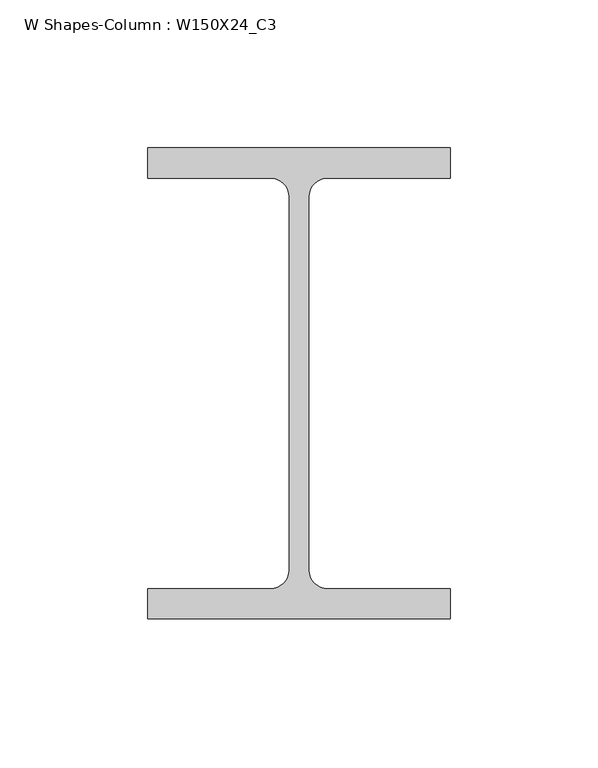
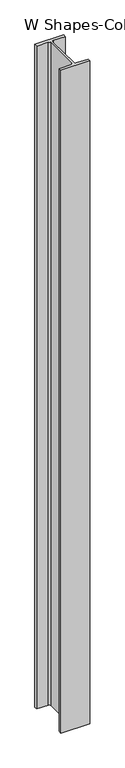
"""IFC4 building model written with IfcOpenShell, lengths in millimetres: column geometry, W Shapes-Column : W150X24_C3."""

from ifc_helpers import new_model, si_unit, point, frame, frame_2d, origin, place, context, project, spatial, polyline, circle_curve, trimmed, segment, composite_curve, outline, extrude, source, transform, mapped, element, save


def w_shapes_column_w150x24_c3_7353ed80(model_context):
    return source(origin(), model_context, "Body", "SweptSolid", [
        extrude(outline(composite_curve([segment(polyline([(51.181, 79.756), (51.181, 69.469), (9.652, 69.469)]), True, "CONTINUOUS"), segment(trimmed(circle_curve(frame_2d((9.652, 63.119)), 6.35), [point((9.652, 69.469))], [point((3.302, 63.119))], True, "CARTESIAN"), True, "CONTINUOUS"), segment(polyline([(3.302, 63.119), (3.302, -63.119)]), True, "CONTINUOUS"), segment(trimmed(circle_curve(frame_2d((9.652, -63.119)), 6.35), [point((3.302, -63.119))], [point((9.652, -69.469))], True, "CARTESIAN"), True, "CONTINUOUS"), segment(polyline([(9.652, -69.469), (51.181, -69.469), (51.181, -79.756), (-51.181, -79.756), (-51.181, -69.469), (-9.652, -69.469)]), True, "CONTINUOUS"), segment(trimmed(circle_curve(frame_2d((-9.652, -63.119)), 6.35), [point((-9.652, -69.469))], [point((-3.302, -63.119))], True, "CARTESIAN"), True, "CONTINUOUS"), segment(polyline([(-3.302, -63.119), (-3.302, 63.119)]), True, "CONTINUOUS"), segment(trimmed(circle_curve(frame_2d((-9.652, 63.119)), 6.35), [point((-3.302, 63.119))], [point((-9.652, 69.469))], True, "CARTESIAN"), True, "CONTINUOUS"), segment(polyline([(-9.652, 69.469), (-51.181, 69.469), (-51.181, 79.756), (51.181, 79.756)]), True, "CONTINUOUS")], self_intersect=False)), frame((0.0, 0.0, 6546.0), z_axis=(0.0, 0.0, 1.0), x_axis=(1.0, 0.0, 0.0)), (0.0, 0.0, 1.0), 2484.0),
    ])


if __name__ == "__main__":
    model = new_model("IFC4")
    model_context = context("Model", 3, world=origin())
    ifc_project = project(units=[si_unit("LENGTHUNIT", "METRE", prefix="MILLI")], contexts=[model_context])
    site = spatial("IfcSite", under=ifc_project)
    building = spatial("IfcBuilding", under=site)
    placement = place(None, origin())
    w_shapes_column_w150x24_c3_shape = w_shapes_column_w150x24_c3_7353ed80(model_context)
    element("IfcColumn", 1, ObjectType="W Shapes-Column : W150X24_C3", at=placement, inside=building, context=model_context, shape_type="MappedRepresentation", body=[
        mapped(w_shapes_column_w150x24_c3_shape, transform((0.0, 0.0, 0.0), x_axis=(1.0, 0.0, 0.0), y_axis=(0.0, 1.0, 0.0), z_axis=(0.0, 0.0, 1.0))),
    ])
    save(model, "model.ifc")

# Revit data of these elements
# Type "W Shapes-Column : W150X24_C3"
#   Section Name Key = "W6x16"
#   Assembly Code = "B10"
#   Width = 10.2362 cm
#   Web Thickness = 0.6604 cm
#   Web Fillet = 0.635 cm
#   Warping Constant = 10258.1 cm⁶
#   Torsional Moment of Inertia = 9.28196 cm⁴
#   Section Area = 30.5806 cm²
#   Plastic Modulus weak axis = 55.5521 cm³
#   Plastic Modulus strong axis = 191.729 cm³
#   Perimeter = 0.704088 m²/m
#   Nominal Weight = 23.8106 kgf/m
#   Moment of Inertia weak axis = 184.391 cm⁴
#   Moment of Inertia strong axis = 1336.10 cm⁴
#   Height = 15.9512 cm
#   Flange Thickness = 1.0287 cm
#   Elastic Modulus weak axis = 36.0515 cm³
#   Elastic Modulus strong axis = 167.148 cm³
#   Clear Web Height = 19.05 cm
#   Centroid Vertical = 7.9756 cm
#   Centroid Horizontal = 5.1181 cm
#   Bolt Spacing = 5.715 cm
#   Structural Material [instance default] = Steel ASTM A992
#   Principal Axes Angle = 0
# Element 1 (IfcColumn, "W Shapes-Column : W150X24_C3")
#   Structural Material = none
# Materials
#   "Steel ASTM A992": class "Metal", colour RGB 199 199 199, transparency 0, Description = "Structural steel 50ksi", Cost = 0
